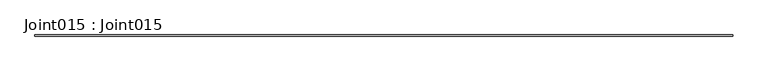
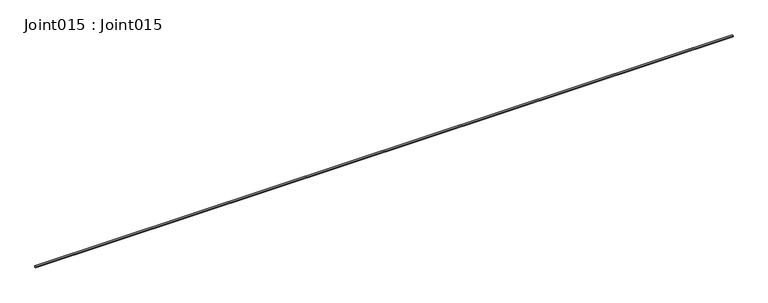
"""IFC4 building model written with IfcOpenShell, lengths in millimetres: proxy geometry, Joint015 : Joint015."""

from ifc_helpers import new_model, si_unit, point, frame, frame_2d, origin, place, context, project, spatial, polyline, circle_curve, trimmed, segment, composite_curve, outline, extrude, source, transform, mapped, element, save


def joint015_joint015_baea0890(model_context):
    return source(origin(), model_context, "Body", "SweptSolid", [
        extrude(outline(composite_curve([segment(polyline([(-4625.5194659, 39007.1389662), (-4625.5194659, 39003.2209974)]), True, "CONTINUOUS"), segment(trimmed(circle_curve(frame_2d((-4627.1177979, 38998.0491224)), 5.4132205), [point((-4625.5194659, 39003.2209974))], [point((-4628.71613, 39003.2209974))], True, "CARTESIAN"), True, "CONTINUOUS"), segment(polyline([(-4628.71613, 39003.2209974), (-4628.71613, 39007.1389662)]), True, "CONTINUOUS"), segment(trimmed(circle_curve(frame_2d((-4627.1177979, 39001.9670912)), 5.4132205), [point((-4628.71613, 39007.1389662))], [point((-4625.5194659, 39007.1389662))], False, "CARTESIAN"), True, "CONTINUOUS")], self_intersect=False)), frame((12383.0178845, 0.0, 0.0), z_axis=(1.0, 0.0, 0.0), x_axis=(0.0, 1.0, 0.0)), (0.0, 0.0, 1.0), 2000.0),
    ])


if __name__ == "__main__":
    model = new_model("IFC4")
    model_context = context("Model", 3, world=origin())
    ifc_project = project(units=[si_unit("LENGTHUNIT", "METRE", prefix="MILLI")], contexts=[model_context])
    site = spatial("IfcSite", under=ifc_project)
    building = spatial("IfcBuilding", under=site)
    placement = place(None, origin())
    joint015_joint015_shape = joint015_joint015_baea0890(model_context)
    element("IfcBuildingElementProxy", 1, Name="Joint015 : Joint015", ObjectType="Joint015 : Joint015", at=placement, inside=building, context=model_context, shape_type="MappedRepresentation", body=[
        mapped(joint015_joint015_shape, transform((0.0, 0.0, 0.0), x_axis=(1.0, 0.0, 0.0), y_axis=(0.0, 1.0, 0.0), z_axis=(0.0, 0.0, 1.0))),
    ])
    save(model, "model.ifc")

# Revit data of these elements
# Type "Joint015 : Joint015"
#   NameOverride = "Joint015"
# Element 1 (IfcBuildingElementProxy, "Joint015 : Joint015")
#   Materials on its faces: "SILICON JOINT"
# Materials
#   "SILICON JOINT": class "Unassigned", colour RGB 150 184 127, transparency 0
